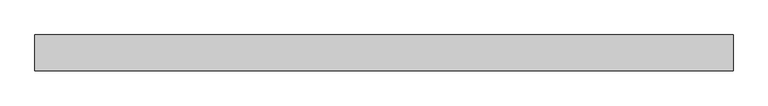
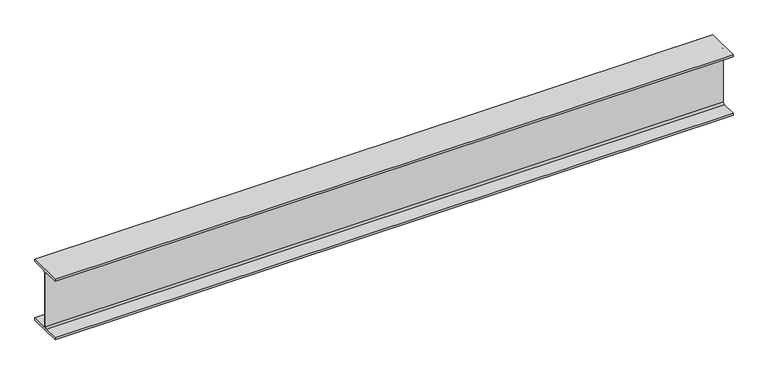
"""IFC4 building model written with IfcOpenShell, lengths in millimetres: beam geometry, Old_Steel Beam_H-KSD3502 : H_SB_ASB_H-200×200x8x12."""

from ifc_helpers import new_model, si_unit, point, frame, frame_2d, origin, place, context, project, spatial, polyline, circle_curve, trimmed, segment, composite_curve, outline, extrude, source, transform, mapped, element, save


def beam_afcd2804(model_context):
    return source(origin(), model_context, "Body", "SweptSolid", [
        extrude(outline(composite_curve([segment(polyline([(82.5, -141.5), (82.5, -151.7), (-82.5, -151.7), (-82.5, -141.5), (-11.9, -141.5)]), True, "CONTINUOUS"), segment(trimmed(circle_curve(frame_2d((-11.9, -132.6)), 8.9), [point((-11.9, -141.5))], [point((-3.0, -132.6))], True, "CARTESIAN"), True, "CONTINUOUS"), segment(polyline([(-3.0, -132.6), (-3.0, 132.6)]), True, "CONTINUOUS"), segment(trimmed(circle_curve(frame_2d((-11.9, 132.6)), 8.9), [point((-3.0, 132.6))], [point((-11.9, 141.5))], True, "CARTESIAN"), True, "CONTINUOUS"), segment(polyline([(-11.9, 141.5), (-82.5, 141.5), (-82.5, 151.7), (82.5, 151.7), (82.5, 141.5), (11.9, 141.5)]), True, "CONTINUOUS"), segment(trimmed(circle_curve(frame_2d((11.9, 132.6)), 8.9), [point((11.9, 141.5))], [point((3.0, 132.6))], True, "CARTESIAN"), True, "CONTINUOUS"), segment(polyline([(3.0, 132.6), (3.0, -132.6)]), True, "CONTINUOUS"), segment(trimmed(circle_curve(frame_2d((11.9, -132.6)), 8.9), [point((3.0, -132.6))], [point((11.9, -141.5))], True, "CARTESIAN"), True, "CONTINUOUS"), segment(polyline([(11.9, -141.5), (82.5, -141.5)]), True, "CONTINUOUS")], self_intersect=False)), frame((-1397.3342488, 0.0, 0.0), z_axis=(1.0, 0.0, 0.0), x_axis=(0.0, 1.0, 0.0)), (0.0, 0.0, 1.0), 3214.0854479),
    ])


if __name__ == "__main__":
    model = new_model("IFC4")
    model_context = context("Model", 3, world=origin())
    ifc_project = project(units=[si_unit("LENGTHUNIT", "METRE", prefix="MILLI")], contexts=[model_context])
    site = spatial("IfcSite", under=ifc_project)
    building = spatial("IfcBuilding", under=site)
    placement = place(None, origin())
    beam_shape = beam_afcd2804(model_context)
    element("IfcBeam", 1, ObjectType="Old_Steel Beam_H-KSD3502 : H_SB_ASB_H-200×200x8x12", at=placement, inside=building, context=model_context, shape_type="MappedRepresentation", body=[
        mapped(beam_shape, transform((0.0, 0.0, 0.0), x_axis=(1.0, 0.0, 0.0), y_axis=(0.0, 1.0, 0.0), z_axis=(0.0, 0.0, 1.0))),
    ])
    save(model, "model.ifc")

# Revit data of these elements
# Type "Old_Steel Beam_H-KSD3502 : H_SB_ASB_H-200×200x8x12"
#   Width = 20.0 cm
#   Web Thickness = 0.8 cm
#   Web Fillet = 1.3 cm
#   Warping Constant = 141376.0 cm⁶
#   Torsional Moment of Inertia = 26.2485 cm⁴
#   Torsional Modulus = 1.0 cm³
#   Section Area = 63.53 cm²
#   Plastic Modulus weak axis = 244.0 cm³
#   Plastic Modulus strong axis = 525.0 cm³
#   Perimeter = 1.16 m²/m
#   Nominal Weight = 49.90 kgf/m
#   Moment of Inertia weak axis = 1600.00 cm⁴
#   Moment of Inertia strong axis = 4720.00 cm⁴
#   Height = 20.0 cm
#   Flange Thickness = 1.2 cm
#   Elastic Modulus weak axis = 160.0 cm³
#   Elastic Modulus strong axis = 472.0 cm³
#   Centroid Vertical = 10.0 cm
#   Centroid Horizontal = 10.0 cm
#   Length [instance default] = 1.5240 m
#   Structural Material [instance default] = Steel, 45-345
#   Assembly Code = ""
# Element 1 (IfcBeam, "Old_Steel Beam_H-KSD3502 : H_SB_ASB_H-200×200x8x12")
#   Structural Material = none
# Materials
#   "Steel, 45-345": class "Metal", colour RGB 189 187 185, transparency 0, Description = "Steel 345 MPa", Cost = 0
